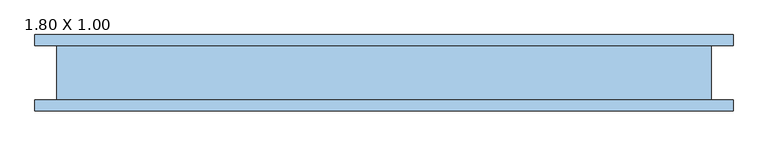
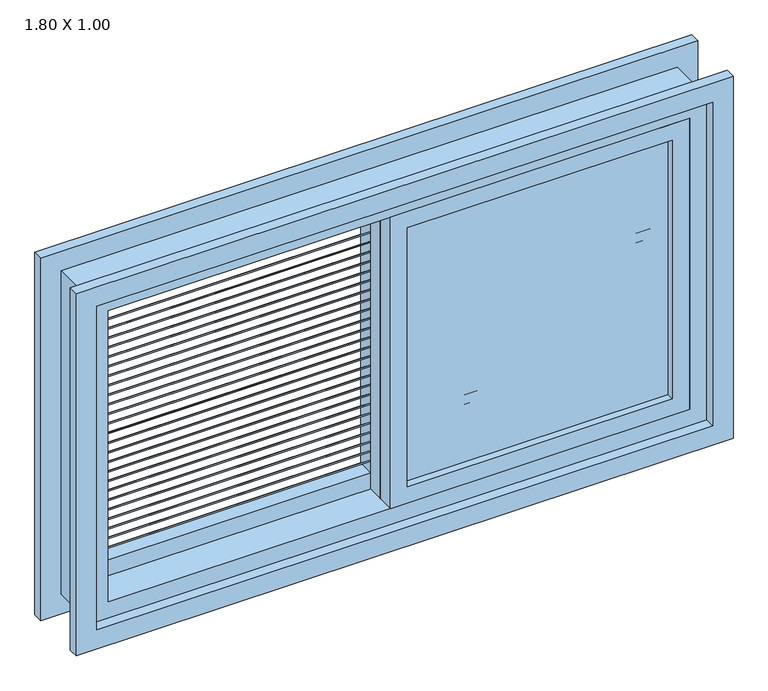
"""IFC4 building model written with IfcOpenShell, lengths in millimetres: window geometry, JANELA_DE_CORRER_3 FOLHAS_VENEZIANA_VIDRO : 1.80 X 1.00."""

from ifc_helpers import new_model, si_unit, frame, origin, place, context, project, spatial, polyline, outline, extrude, source, transform, mapped, element, save


def window_1_80_x_1_00_6147d50d(model_context):
    return source(origin(), model_context, "Body", "SweptSolid", [
        extrude(outline(polyline([(20.0, 1835.5769231), (-25.0, 1870.5769231), (-20.0, 1870.5769231), (25.0, 1835.5769231), (20.0, 1835.5769231)])), frame((25.0, 0.0, 0.0), z_axis=(1.0, 0.0, 0.0), x_axis=(0.0, 1.0, 0.0)), (0.0, 0.0, 1.0), 775.0),
        extrude(outline(polyline([(20.0, 1806.1538462), (-25.0, 1841.1538462), (-20.0, 1841.1538462), (25.0, 1806.1538462), (20.0, 1806.1538462)])), frame((25.0, 0.0, 0.0), z_axis=(1.0, 0.0, 0.0), x_axis=(0.0, 1.0, 0.0)), (0.0, 0.0, 1.0), 775.0),
        extrude(outline(polyline([(20.0, 1776.7307692), (-25.0, 1811.7307692), (-20.0, 1811.7307692), (25.0, 1776.7307692), (20.0, 1776.7307692)])), frame((25.0, 0.0, 0.0), z_axis=(1.0, 0.0, 0.0), x_axis=(0.0, 1.0, 0.0)), (0.0, 0.0, 1.0), 775.0),
        extrude(outline(polyline([(20.0, 1747.3076923), (-25.0, 1782.3076923), (-20.0, 1782.3076923), (25.0, 1747.3076923), (20.0, 1747.3076923)])), frame((25.0, 0.0, 0.0), z_axis=(1.0, 0.0, 0.0), x_axis=(0.0, 1.0, 0.0)), (0.0, 0.0, 1.0), 775.0),
        extrude(outline(polyline([(20.0, 1717.8846154), (-25.0, 1752.8846154), (-20.0, 1752.8846154), (25.0, 1717.8846154), (20.0, 1717.8846154)])), frame((25.0, 0.0, 0.0), z_axis=(1.0, 0.0, 0.0), x_axis=(0.0, 1.0, 0.0)), (0.0, 0.0, 1.0), 775.0),
        extrude(outline(polyline([(20.0, 1688.4615385), (-25.0, 1723.4615385), (-20.0, 1723.4615385), (25.0, 1688.4615385), (20.0, 1688.4615385)])), frame((25.0, 0.0, 0.0), z_axis=(1.0, 0.0, 0.0), x_axis=(0.0, 1.0, 0.0)), (0.0, 0.0, 1.0), 775.0),
        extrude(outline(polyline([(20.0, 1659.0384615), (-25.0, 1694.0384615), (-20.0, 1694.0384615), (25.0, 1659.0384615), (20.0, 1659.0384615)])), frame((25.0, 0.0, 0.0), z_axis=(1.0, 0.0, 0.0), x_axis=(0.0, 1.0, 0.0)), (0.0, 0.0, 1.0), 775.0),
        extrude(outline(polyline([(20.0, 1629.6153846), (-25.0, 1664.6153846), (-20.0, 1664.6153846), (25.0, 1629.6153846), (20.0, 1629.6153846)])), frame((25.0, 0.0, 0.0), z_axis=(1.0, 0.0, 0.0), x_axis=(0.0, 1.0, 0.0)), (0.0, 0.0, 1.0), 775.0),
        extrude(outline(polyline([(20.0, 1600.1923077), (-25.0, 1635.1923077), (-20.0, 1635.1923077), (25.0, 1600.1923077), (20.0, 1600.1923077)])), frame((25.0, 0.0, 0.0), z_axis=(1.0, 0.0, 0.0), x_axis=(0.0, 1.0, 0.0)), (0.0, 0.0, 1.0), 775.0),
        extrude(outline(polyline([(20.0, 1570.7692308), (-25.0, 1605.7692308), (-20.0, 1605.7692308), (25.0, 1570.7692308), (20.0, 1570.7692308)])), frame((25.0, 0.0, 0.0), z_axis=(1.0, 0.0, 0.0), x_axis=(0.0, 1.0, 0.0)), (0.0, 0.0, 1.0), 775.0),
        extrude(outline(polyline([(20.0, 1541.3461538), (-25.0, 1576.3461538), (-20.0, 1576.3461538), (25.0, 1541.3461538), (20.0, 1541.3461538)])), frame((25.0, 0.0, 0.0), z_axis=(1.0, 0.0, 0.0), x_axis=(0.0, 1.0, 0.0)), (0.0, 0.0, 1.0), 775.0),
        extrude(outline(polyline([(20.0, 1511.9230769), (-25.0, 1546.9230769), (-20.0, 1546.9230769), (25.0, 1511.9230769), (20.0, 1511.9230769)])), frame((25.0, 0.0, 0.0), z_axis=(1.0, 0.0, 0.0), x_axis=(0.0, 1.0, 0.0)), (0.0, 0.0, 1.0), 775.0),
        extrude(outline(polyline([(20.0, 1482.5), (-25.0, 1517.5), (-20.0, 1517.5), (25.0, 1482.5), (20.0, 1482.5)])), frame((25.0, 0.0, 0.0), z_axis=(1.0, 0.0, 0.0), x_axis=(0.0, 1.0, 0.0)), (0.0, 0.0, 1.0), 775.0),
        extrude(outline(polyline([(20.0, 1453.0769231), (-25.0, 1488.0769231), (-20.0, 1488.0769231), (25.0, 1453.0769231), (20.0, 1453.0769231)])), frame((25.0, 0.0, 0.0), z_axis=(1.0, 0.0, 0.0), x_axis=(0.0, 1.0, 0.0)), (0.0, 0.0, 1.0), 775.0),
        extrude(outline(polyline([(20.0, 1423.6538462), (-25.0, 1458.6538462), (-20.0, 1458.6538462), (25.0, 1423.6538462), (20.0, 1423.6538462)])), frame((25.0, 0.0, 0.0), z_axis=(1.0, 0.0, 0.0), x_axis=(0.0, 1.0, 0.0)), (0.0, 0.0, 1.0), 775.0),
        extrude(outline(polyline([(20.0, 1394.2307692), (-25.0, 1429.2307692), (-20.0, 1429.2307692), (25.0, 1394.2307692), (20.0, 1394.2307692)])), frame((25.0, 0.0, 0.0), z_axis=(1.0, 0.0, 0.0), x_axis=(0.0, 1.0, 0.0)), (0.0, 0.0, 1.0), 775.0),
        extrude(outline(polyline([(20.0, 1364.8076923), (-25.0, 1399.8076923), (-20.0, 1399.8076923), (25.0, 1364.8076923), (20.0, 1364.8076923)])), frame((25.0, 0.0, 0.0), z_axis=(1.0, 0.0, 0.0), x_axis=(0.0, 1.0, 0.0)), (0.0, 0.0, 1.0), 775.0),
        extrude(outline(polyline([(20.0, 1335.3846154), (-25.0, 1370.3846154), (-20.0, 1370.3846154), (25.0, 1335.3846154), (20.0, 1335.3846154)])), frame((25.0, 0.0, 0.0), z_axis=(1.0, 0.0, 0.0), x_axis=(0.0, 1.0, 0.0)), (0.0, 0.0, 1.0), 775.0),
        extrude(outline(polyline([(20.0, 1305.9615385), (-25.0, 1340.9615385), (-20.0, 1340.9615385), (25.0, 1305.9615385), (20.0, 1305.9615385)])), frame((25.0, 0.0, 0.0), z_axis=(1.0, 0.0, 0.0), x_axis=(0.0, 1.0, 0.0)), (0.0, 0.0, 1.0), 775.0),
        extrude(outline(polyline([(20.0, 1276.5384615), (-25.0, 1311.5384615), (-20.0, 1311.5384615), (25.0, 1276.5384615), (20.0, 1276.5384615)])), frame((25.0, 0.0, 0.0), z_axis=(1.0, 0.0, 0.0), x_axis=(0.0, 1.0, 0.0)), (0.0, 0.0, 1.0), 775.0),
        extrude(outline(polyline([(20.0, 1247.1153846), (-25.0, 1282.1153846), (-20.0, 1282.1153846), (25.0, 1247.1153846), (20.0, 1247.1153846)])), frame((25.0, 0.0, 0.0), z_axis=(1.0, 0.0, 0.0), x_axis=(0.0, 1.0, 0.0)), (0.0, 0.0, 1.0), 775.0),
        extrude(outline(polyline([(20.0, 1217.6923077), (-25.0, 1252.6923077), (-20.0, 1252.6923077), (25.0, 1217.6923077), (20.0, 1217.6923077)])), frame((25.0, 0.0, 0.0), z_axis=(1.0, 0.0, 0.0), x_axis=(0.0, 1.0, 0.0)), (0.0, 0.0, 1.0), 775.0),
        extrude(outline(polyline([(20.0, 1188.2692308), (-25.0, 1223.2692308), (-20.0, 1223.2692308), (25.0, 1188.2692308), (20.0, 1188.2692308)])), frame((25.0, 0.0, 0.0), z_axis=(1.0, 0.0, 0.0), x_axis=(0.0, 1.0, 0.0)), (0.0, 0.0, 1.0), 775.0),
        extrude(outline(polyline([(20.0, 1158.8461538), (-25.0, 1193.8461538), (-20.0, 1193.8461538), (25.0, 1158.8461538), (20.0, 1158.8461538)])), frame((25.0, 0.0, 0.0), z_axis=(1.0, 0.0, 0.0), x_axis=(0.0, 1.0, 0.0)), (0.0, 0.0, 1.0), 775.0),
        extrude(outline(polyline([(20.0, 1129.4230769), (-25.0, 1164.4230769), (-20.0, 1164.4230769), (25.0, 1129.4230769), (20.0, 1129.4230769)])), frame((25.0, 0.0, 0.0), z_axis=(1.0, 0.0, 0.0), x_axis=(0.0, 1.0, 0.0)), (0.0, 0.0, 1.0), 775.0),
        extrude(outline(polyline([(20.0, 1865.0), (-25.0, 1900.0), (-20.0, 1900.0), (25.0, 1865.0), (20.0, 1865.0)])), frame((25.0, 0.0, 0.0), z_axis=(1.0, 0.0, 0.0), x_axis=(0.0, 1.0, 0.0)), (0.0, 0.0, 1.0), 775.0),
        extrude(outline(polyline([(20.0, 1100.0), (-25.0, 1135.0), (-20.0, 1135.0), (25.0, 1100.0), (20.0, 1100.0)])), frame((25.0, 0.0, 0.0), z_axis=(1.0, 0.0, 0.0), x_axis=(0.0, 1.0, 0.0)), (0.0, 0.0, 1.0), 775.0),
        extrude(outline(polyline([(1950.0, 850.0), (1950.0, -25.0), (1050.0, -25.0), (1050.0, 850.0), (1950.0, 850.0)]), holes=[polyline([(1900.0, 800.0), (1100.0, 800.0), (1100.0, 25.0), (1900.0, 25.0), (1900.0, 800.0)])]), frame((0.0, -25.0, 0.0), z_axis=(0.0, 1.0, 0.0), x_axis=(0.0, 0.0, 1.0)), (0.0, 0.0, 1.0), 50.0),
        extrude(outline(polyline([(800.0, -47.5), (800.0, -52.5), (25.0, -52.5), (25.0, -47.5), (800.0, -47.5)])), frame((0.0, 0.0, 1100.0), z_axis=(0.0, 0.0, 1.0), x_axis=(1.0, 0.0, 0.0)), (0.0, 0.0, 1.0), 800.0),
        extrude(outline(polyline([(1950.0, 850.0), (1950.0, -25.0), (1050.0, -25.0), (1050.0, 850.0), (1950.0, 850.0)]), holes=[polyline([(1900.0, 800.0), (1100.0, 800.0), (1100.0, 25.0), (1900.0, 25.0), (1900.0, 800.0)])]), frame((0.0, -75.0, 0.0), z_axis=(0.0, 1.0, 0.0), x_axis=(0.0, 0.0, 1.0)), (0.0, 0.0, 1.0), 50.0),
        extrude(outline(polyline([(70.0, 1835.5769231), (25.0, 1870.5769231), (30.0, 1870.5769231), (75.0, 1835.5769231), (70.0, 1835.5769231)])), frame((-800.0, 0.0, 0.0), z_axis=(1.0, 0.0, 0.0), x_axis=(0.0, 1.0, 0.0)), (0.0, 0.0, 1.0), 775.0),
        extrude(outline(polyline([(70.0, 1806.1538462), (25.0, 1841.1538462), (30.0, 1841.1538462), (75.0, 1806.1538462), (70.0, 1806.1538462)])), frame((-800.0, 0.0, 0.0), z_axis=(1.0, 0.0, 0.0), x_axis=(0.0, 1.0, 0.0)), (0.0, 0.0, 1.0), 775.0),
        extrude(outline(polyline([(70.0, 1776.7307692), (25.0, 1811.7307692), (30.0, 1811.7307692), (75.0, 1776.7307692), (70.0, 1776.7307692)])), frame((-800.0, 0.0, 0.0), z_axis=(1.0, 0.0, 0.0), x_axis=(0.0, 1.0, 0.0)), (0.0, 0.0, 1.0), 775.0),
        extrude(outline(polyline([(70.0, 1747.3076923), (25.0, 1782.3076923), (30.0, 1782.3076923), (75.0, 1747.3076923), (70.0, 1747.3076923)])), frame((-800.0, 0.0, 0.0), z_axis=(1.0, 0.0, 0.0), x_axis=(0.0, 1.0, 0.0)), (0.0, 0.0, 1.0), 775.0),
        extrude(outline(polyline([(70.0, 1717.8846154), (25.0, 1752.8846154), (30.0, 1752.8846154), (75.0, 1717.8846154), (70.0, 1717.8846154)])), frame((-800.0, 0.0, 0.0), z_axis=(1.0, 0.0, 0.0), x_axis=(0.0, 1.0, 0.0)), (0.0, 0.0, 1.0), 775.0),
        extrude(outline(polyline([(70.0, 1688.4615385), (25.0, 1723.4615385), (30.0, 1723.4615385), (75.0, 1688.4615385), (70.0, 1688.4615385)])), frame((-800.0, 0.0, 0.0), z_axis=(1.0, 0.0, 0.0), x_axis=(0.0, 1.0, 0.0)), (0.0, 0.0, 1.0), 775.0),
        extrude(outline(polyline([(70.0, 1659.0384615), (25.0, 1694.0384615), (30.0, 1694.0384615), (75.0, 1659.0384615), (70.0, 1659.0384615)])), frame((-800.0, 0.0, 0.0), z_axis=(1.0, 0.0, 0.0), x_axis=(0.0, 1.0, 0.0)), (0.0, 0.0, 1.0), 775.0),
        extrude(outline(polyline([(70.0, 1629.6153846), (25.0, 1664.6153846), (30.0, 1664.6153846), (75.0, 1629.6153846), (70.0, 1629.6153846)])), frame((-800.0, 0.0, 0.0), z_axis=(1.0, 0.0, 0.0), x_axis=(0.0, 1.0, 0.0)), (0.0, 0.0, 1.0), 775.0),
        extrude(outline(polyline([(70.0, 1600.1923077), (25.0, 1635.1923077), (30.0, 1635.1923077), (75.0, 1600.1923077), (70.0, 1600.1923077)])), frame((-800.0, 0.0, 0.0), z_axis=(1.0, 0.0, 0.0), x_axis=(0.0, 1.0, 0.0)), (0.0, 0.0, 1.0), 775.0),
        extrude(outline(polyline([(70.0, 1570.7692308), (25.0, 1605.7692308), (30.0, 1605.7692308), (75.0, 1570.7692308), (70.0, 1570.7692308)])), frame((-800.0, 0.0, 0.0), z_axis=(1.0, 0.0, 0.0), x_axis=(0.0, 1.0, 0.0)), (0.0, 0.0, 1.0), 775.0),
        extrude(outline(polyline([(70.0, 1541.3461538), (25.0, 1576.3461538), (30.0, 1576.3461538), (75.0, 1541.3461538), (70.0, 1541.3461538)])), frame((-800.0, 0.0, 0.0), z_axis=(1.0, 0.0, 0.0), x_axis=(0.0, 1.0, 0.0)), (0.0, 0.0, 1.0), 775.0),
        extrude(outline(polyline([(70.0, 1511.9230769), (25.0, 1546.9230769), (30.0, 1546.9230769), (75.0, 1511.9230769), (70.0, 1511.9230769)])), frame((-800.0, 0.0, 0.0), z_axis=(1.0, 0.0, 0.0), x_axis=(0.0, 1.0, 0.0)), (0.0, 0.0, 1.0), 775.0),
        extrude(outline(polyline([(70.0, 1482.5), (25.0, 1517.5), (30.0, 1517.5), (75.0, 1482.5), (70.0, 1482.5)])), frame((-800.0, 0.0, 0.0), z_axis=(1.0, 0.0, 0.0), x_axis=(0.0, 1.0, 0.0)), (0.0, 0.0, 1.0), 775.0),
        extrude(outline(polyline([(70.0, 1453.0769231), (25.0, 1488.0769231), (30.0, 1488.0769231), (75.0, 1453.0769231), (70.0, 1453.0769231)])), frame((-800.0, 0.0, 0.0), z_axis=(1.0, 0.0, 0.0), x_axis=(0.0, 1.0, 0.0)), (0.0, 0.0, 1.0), 775.0),
        extrude(outline(polyline([(70.0, 1423.6538462), (25.0, 1458.6538462), (30.0, 1458.6538462), (75.0, 1423.6538462), (70.0, 1423.6538462)])), frame((-800.0, 0.0, 0.0), z_axis=(1.0, 0.0, 0.0), x_axis=(0.0, 1.0, 0.0)), (0.0, 0.0, 1.0), 775.0),
        extrude(outline(polyline([(70.0, 1394.2307692), (25.0, 1429.2307692), (30.0, 1429.2307692), (75.0, 1394.2307692), (70.0, 1394.2307692)])), frame((-800.0, 0.0, 0.0), z_axis=(1.0, 0.0, 0.0), x_axis=(0.0, 1.0, 0.0)), (0.0, 0.0, 1.0), 775.0),
        extrude(outline(polyline([(70.0, 1364.8076923), (25.0, 1399.8076923), (30.0, 1399.8076923), (75.0, 1364.8076923), (70.0, 1364.8076923)])), frame((-800.0, 0.0, 0.0), z_axis=(1.0, 0.0, 0.0), x_axis=(0.0, 1.0, 0.0)), (0.0, 0.0, 1.0), 775.0),
        extrude(outline(polyline([(70.0, 1335.3846154), (25.0, 1370.3846154), (30.0, 1370.3846154), (75.0, 1335.3846154), (70.0, 1335.3846154)])), frame((-800.0, 0.0, 0.0), z_axis=(1.0, 0.0, 0.0), x_axis=(0.0, 1.0, 0.0)), (0.0, 0.0, 1.0), 775.0),
        extrude(outline(polyline([(70.0, 1305.9615385), (25.0, 1340.9615385), (30.0, 1340.9615385), (75.0, 1305.9615385), (70.0, 1305.9615385)])), frame((-800.0, 0.0, 0.0), z_axis=(1.0, 0.0, 0.0), x_axis=(0.0, 1.0, 0.0)), (0.0, 0.0, 1.0), 775.0),
        extrude(outline(polyline([(70.0, 1276.5384615), (25.0, 1311.5384615), (30.0, 1311.5384615), (75.0, 1276.5384615), (70.0, 1276.5384615)])), frame((-800.0, 0.0, 0.0), z_axis=(1.0, 0.0, 0.0), x_axis=(0.0, 1.0, 0.0)), (0.0, 0.0, 1.0), 775.0),
        extrude(outline(polyline([(70.0, 1247.1153846), (25.0, 1282.1153846), (30.0, 1282.1153846), (75.0, 1247.1153846), (70.0, 1247.1153846)])), frame((-800.0, 0.0, 0.0), z_axis=(1.0, 0.0, 0.0), x_axis=(0.0, 1.0, 0.0)), (0.0, 0.0, 1.0), 775.0),
        extrude(outline(polyline([(70.0, 1217.6923077), (25.0, 1252.6923077), (30.0, 1252.6923077), (75.0, 1217.6923077), (70.0, 1217.6923077)])), frame((-800.0, 0.0, 0.0), z_axis=(1.0, 0.0, 0.0), x_axis=(0.0, 1.0, 0.0)), (0.0, 0.0, 1.0), 775.0),
        extrude(outline(polyline([(70.0, 1188.2692308), (25.0, 1223.2692308), (30.0, 1223.2692308), (75.0, 1188.2692308), (70.0, 1188.2692308)])), frame((-800.0, 0.0, 0.0), z_axis=(1.0, 0.0, 0.0), x_axis=(0.0, 1.0, 0.0)), (0.0, 0.0, 1.0), 775.0),
        extrude(outline(polyline([(70.0, 1158.8461538), (25.0, 1193.8461538), (30.0, 1193.8461538), (75.0, 1158.8461538), (70.0, 1158.8461538)])), frame((-800.0, 0.0, 0.0), z_axis=(1.0, 0.0, 0.0), x_axis=(0.0, 1.0, 0.0)), (0.0, 0.0, 1.0), 775.0),
        extrude(outline(polyline([(70.0, 1129.4230769), (25.0, 1164.4230769), (30.0, 1164.4230769), (75.0, 1129.4230769), (70.0, 1129.4230769)])), frame((-800.0, 0.0, 0.0), z_axis=(1.0, 0.0, 0.0), x_axis=(0.0, 1.0, 0.0)), (0.0, 0.0, 1.0), 775.0),
        extrude(outline(polyline([(70.0, 1865.0), (25.0, 1900.0), (30.0, 1900.0), (75.0, 1865.0), (70.0, 1865.0)])), frame((-800.0, 0.0, 0.0), z_axis=(1.0, 0.0, 0.0), x_axis=(0.0, 1.0, 0.0)), (0.0, 0.0, 1.0), 775.0),
        extrude(outline(polyline([(70.0, 1100.0), (25.0, 1135.0), (30.0, 1135.0), (75.0, 1100.0), (70.0, 1100.0)])), frame((-800.0, 0.0, 0.0), z_axis=(1.0, 0.0, 0.0), x_axis=(0.0, 1.0, 0.0)), (0.0, 0.0, 1.0), 775.0),
        extrude(outline(polyline([(1950.0, 25.0), (1950.0, -850.0), (1050.0, -850.0), (1050.0, 25.0), (1950.0, 25.0)]), holes=[polyline([(1900.0, -25.0), (1100.0, -25.0), (1100.0, -800.0), (1900.0, -800.0), (1900.0, -25.0)])]), frame((0.0, 25.0, 0.0), z_axis=(0.0, 1.0, 0.0), x_axis=(0.0, 0.0, 1.0)), (0.0, 0.0, 1.0), 50.0),
        extrude(outline(polyline([(940.0, -960.0), (940.0, 960.0), (2060.0, 960.0), (2060.0, -960.0), (940.0, -960.0)]), holes=[polyline([(1000.0, -900.0), (2000.0, -900.0), (2000.0, 900.0), (1000.0, 900.0), (1000.0, -900.0)])]), frame((0.0, 75.0, 0.0), z_axis=(0.0, 1.0, 0.0), x_axis=(0.0, 0.0, 1.0)), (0.0, 0.0, 1.0), 30.0),
        extrude(outline(polyline([(940.0, -960.0), (940.0, 960.0), (2060.0, 960.0), (2060.0, -960.0), (940.0, -960.0)]), holes=[polyline([(1000.0, -900.0), (2000.0, -900.0), (2000.0, 900.0), (1000.0, 900.0), (1000.0, -900.0)])]), frame((0.0, -105.0, 0.0), z_axis=(0.0, 1.0, 0.0), x_axis=(0.0, 0.0, 1.0)), (0.0, 0.0, 1.0), 30.0),
        extrude(outline(polyline([(1000.0, -900.0), (1000.0, 900.0), (2000.0, 900.0), (2000.0, -900.0), (1000.0, -900.0)]), holes=[polyline([(1950.0, -850.0), (1950.0, 850.0), (1050.0, 850.0), (1050.0, -850.0), (1950.0, -850.0)])]), frame((0.0, -75.0, 0.0), z_axis=(0.0, 1.0, 0.0), x_axis=(0.0, 0.0, 1.0)), (0.0, 0.0, 1.0), 150.0),
    ])


if __name__ == "__main__":
    model = new_model("IFC4")
    model_context = context("Model", 3, world=origin())
    ifc_project = project(units=[si_unit("LENGTHUNIT", "METRE", prefix="MILLI")], contexts=[model_context])
    site = spatial("IfcSite", under=ifc_project)
    building = spatial("IfcBuilding", under=site)
    placement = place(None, origin())
    window_1_80_x_1_00_shape = window_1_80_x_1_00_6147d50d(model_context)
    element("IfcWindow", 1, ObjectType="JANELA_DE_CORRER_3 FOLHAS_VENEZIANA_VIDRO : 1.80 X 1.00", at=placement, inside=building, context=model_context, shape_type="MappedRepresentation", body=[
        mapped(window_1_80_x_1_00_shape, transform((0.0, 0.0, 0.0), x_axis=(1.0, 0.0, 0.0), y_axis=(0.0, 1.0, 0.0), z_axis=(0.0, 0.0, 1.0))),
    ])
    save(model, "model.ifc")

# Revit data of these elements
# Type "JANELA_DE_CORRER_3 FOLHAS_VENEZIANA_VIDRO : 1.80 X 1.00"
#   Type Mark = "J17"
#   Analytic Construction = "<Nenhum>"
#   Largura moldura = 0.06 m
#   Largura janela = 1.70 m
#   Largura esquadria = 0.05 m
#   Largura do painel = 0.875 m
#   Largura da moldura do painel = 0.05 m
#   Espessura esquadria = 0.15 m
#   Espessura painel = 0.05 m
#   Espessura moldura = 0.03 m
#   Altura janela = 0.90 m
#   Height = 1.00 m
#   Altura-padrão do peitoril = 1.00 m
#   Width = 1.80 m
#   Moldura interna [instance default] = yes
#   Moldura externa [instance default] = yes
#   Tipo de vidro = .VIDRO
#   Material moldura = .ALUMÍNIO COM PINTURA ELETROSTÁTICA BRANCA
#   Material da esquadria = .ALUMÍNIO COM PINTURA ELETROSTÁTICA BRANCA
#   Wall Closure = (empty or 0)
# Element 1 (IfcWindow, "JANELA_DE_CORRER_3 FOLHAS_VENEZIANA_VIDRO : 1.80 X 1.00")
#   Materials on its faces: ".ALUMÍNIO COM PINTURA ELETROSTÁTICA BRANCA", ".VIDRO"
# Materials
#   ".VIDRO": class "Genérico", colour RGB 198 236 255, transparency 0.95, Cost = 0
#   ".ALUMÍNIO COM PINTURA ELETROSTÁTICA BRANCA": class "CC_METAIS", colour RGB 241 241 241, transparency 0, Cost = 0
